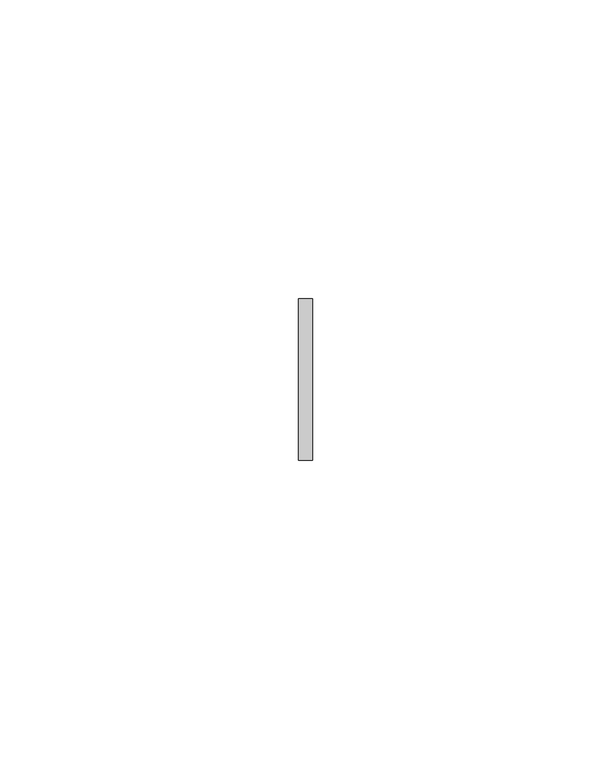
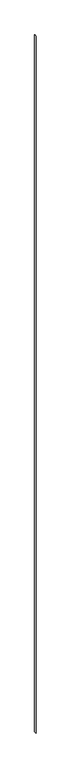
"""IFC4 building model written with IfcOpenShell, lengths in millimetres: proxy geometry, Generic Models 2:Generic Models 2:310765:Generic Models 2:310765 : Generic Models 2:Generic Models 2:310765:71 : Generic Models 2:Generic Models 2:310765:Generic Models 2:310765 : Generic Models 2:Generic Models 2:310765:300385."""

from ifc_helpers import new_model, si_unit, origin, origin_with_axes, place, context, project, spatial, polyline, outline, extrude, source, transform, mapped, element, save


def generic_models_e3b5e946(model_context):
    return source(origin(), model_context, "Body", "SweptSolid", [
        extrude(outline(polyline([(667547.3117239, -564680.4915363), (667549.5995663, -564680.4915363), (667549.5995663, -564707.4790363), (667547.3117239, -564707.4790363), (667547.3117239, -564680.4915363)])), origin_with_axes(), (0.0, 0.0, 1.0), 8555.7679991),
    ])


if __name__ == "__main__":
    model = new_model("IFC4")
    model_context = context("Model", 3, world=origin())
    ifc_project = project(units=[si_unit("LENGTHUNIT", "METRE", prefix="MILLI")], contexts=[model_context])
    site = spatial("IfcSite", under=ifc_project)
    building = spatial("IfcBuilding", under=site)
    placement = place(None, origin())
    generic_models_shape = generic_models_e3b5e946(model_context)
    element("IfcBuildingElementProxy", 1, Name="Generic Models 2:Generic Models 2:310765:Generic Models 2:310765 : Generic Models 2:Generic Models 2:310765:71 : Generic Models 2:Generic Models 2:310765:Generic Models 2:310765 : Generic Models 2:Generic Models 2:310765:300385", ObjectType="Generic Models 2:Generic Models 2:310765:Generic Models 2:310765 : Generic Models 2:Generic Models 2:310765:71 : Generic Models 2:Generic Models 2:310765:Generic Models 2:310765 : Generic Models 2:Generic Models 2:310765:300385", at=placement, inside=building, context=model_context, shape_type="MappedRepresentation", body=[
        mapped(generic_models_shape, transform((0.0, 0.0, 0.0), x_axis=(1.0, 0.0, 0.0), y_axis=(0.0, 1.0, 0.0), z_axis=(0.0, 0.0, 1.0))),
    ])
    save(model, "model.ifc")

# Revit data of these elements
# Type "Generic Models 2:Generic Models 2:310765:Generic Models 2:310765 : Generic Models 2:Generic Models 2:310765:71 : Generic Models 2:Generic Models 2:310765:Generic Models 2:310765 : Generic Models 2:Generic Models 2:310765:300385"
#   NameOverride = "Generic Models 2:Generic Models 2:310765:Generic Models 2:310765 : Generic Models 2:Generic Models 2:310765:300385"
#   ObjectTypeOverride = "Generic Models 2:310765 : Generic Models 2:Generic Models 2:310765"
#   Reference = "Generic Models 2"
#   Tag = "300385"
# Element 1 (IfcBuildingElementProxy, "Generic Models 2:Generic Models 2:310765:Generic Models 2:310765 : Generic Models 2:Generic Models 2:310765:71 : Generic Models 2:Generic Models 2:310765:Generic Models 2:310765 : Generic Models 2:Generic Models 2:310765:300385")
#   Materials on its faces: "COMPRESSIBE THERMAL GASKET SANDWICHED BETWEEN METAL COMPONENTS"
# Materials
#   "COMPRESSIBE THERMAL GASKET SANDWICHED BETWEEN METAL COMPONENTS": class "Unassigned", colour RGB 58 208 21, transparency 0, Cost = 0
